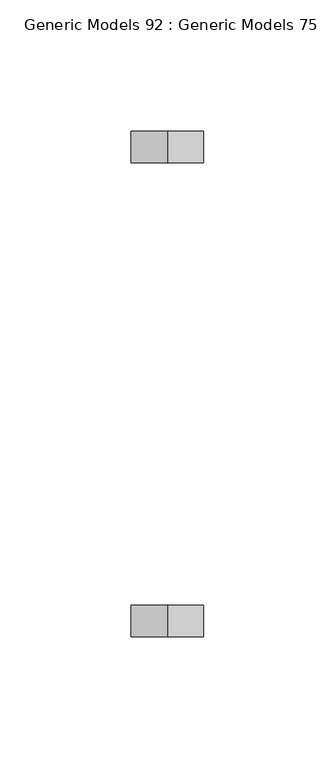
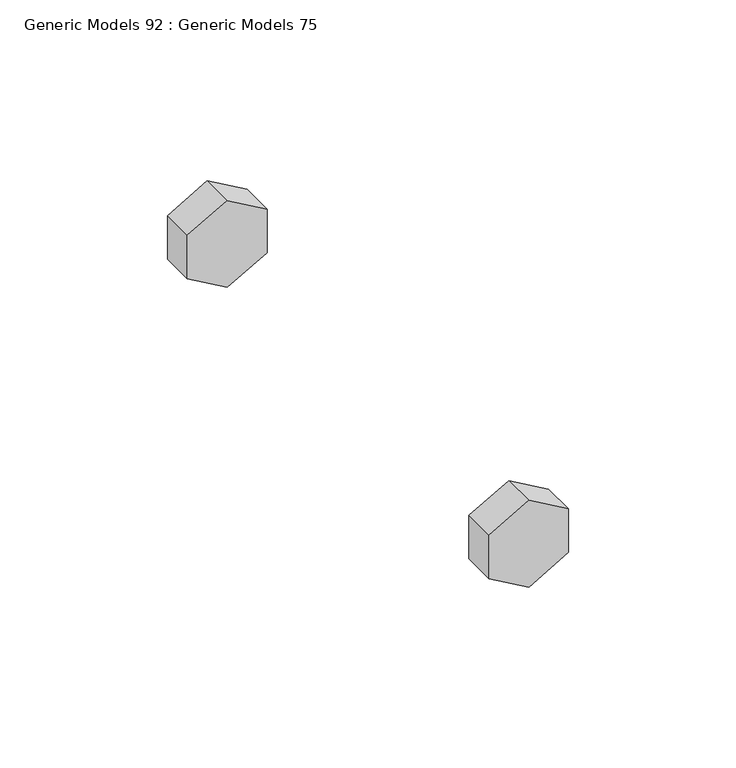
"""IFC4 building model written with IfcOpenShell, lengths in millimetres: proxy geometry, Generic Models 92 : Generic Models 75."""

from ifc_helpers import new_model, si_unit, frame, origin, place, context, project, spatial, polyline, outline, extrude, source, transform, mapped, element, save


def generic_models_92_generic_models_75_5f54ca5c(model_context):
    return source(origin(), model_context, "Body", "SweptSolid", [
        extrude(outline(polyline([(269374.7462802, 31974.4067029), (269358.9097067, 31974.4067029), (269350.99142, 31988.1215778), (269358.9097067, 32001.8364528), (269374.7462802, 32001.8364528), (269382.664567, 31988.1215778), (269374.7462802, 31974.4067029)])), frame((0.0, 36491.5582942, 0.0), z_axis=(0.0, 1.0, 0.0), x_axis=(0.0, 0.0, 1.0)), (0.0, 0.0, 1.0), 11.90625),
        extrude(outline(polyline([(269374.7462802, 31974.4067029), (269358.9097067, 31974.4067029), (269350.99142, 31988.1215778), (269358.9097067, 32001.8364528), (269374.7462802, 32001.8364528), (269382.664567, 31988.1215778), (269374.7462802, 31974.4067029)])), frame((0.0, 36311.3770442, 0.0), z_axis=(0.0, 1.0, 0.0), x_axis=(0.0, 0.0, 1.0)), (0.0, 0.0, 1.0), 11.90625),
    ])


if __name__ == "__main__":
    model = new_model("IFC4")
    model_context = context("Model", 3, world=origin())
    ifc_project = project(units=[si_unit("LENGTHUNIT", "METRE", prefix="MILLI")], contexts=[model_context])
    site = spatial("IfcSite", under=ifc_project)
    building = spatial("IfcBuilding", under=site)
    placement = place(None, origin())
    generic_models_92_generic_models_75_shape = generic_models_92_generic_models_75_5f54ca5c(model_context)
    element("IfcBuildingElementProxy", 1, Name="Generic Models 92 : Generic Models 75", ObjectType="Generic Models 92 : Generic Models 75", at=placement, inside=building, context=model_context, shape_type="MappedRepresentation", body=[
        mapped(generic_models_92_generic_models_75_shape, transform((0.0, 0.0, 0.0), x_axis=(1.0, 0.0, 0.0), y_axis=(0.0, 1.0, 0.0), z_axis=(0.0, 0.0, 1.0))),
    ])
    save(model, "model.ifc")

# Revit data of these elements
# Element 1 (IfcBuildingElementProxy, "Generic Models 92 : Generic Models 75")
#   Materials on its faces: "3/4\" GALV. THRU BOLTS"
# Materials
#   "3/4\" GALV. THRU BOLTS": class "Generic", colour RGB 105 69 171, transparency 0, Cost = 0
